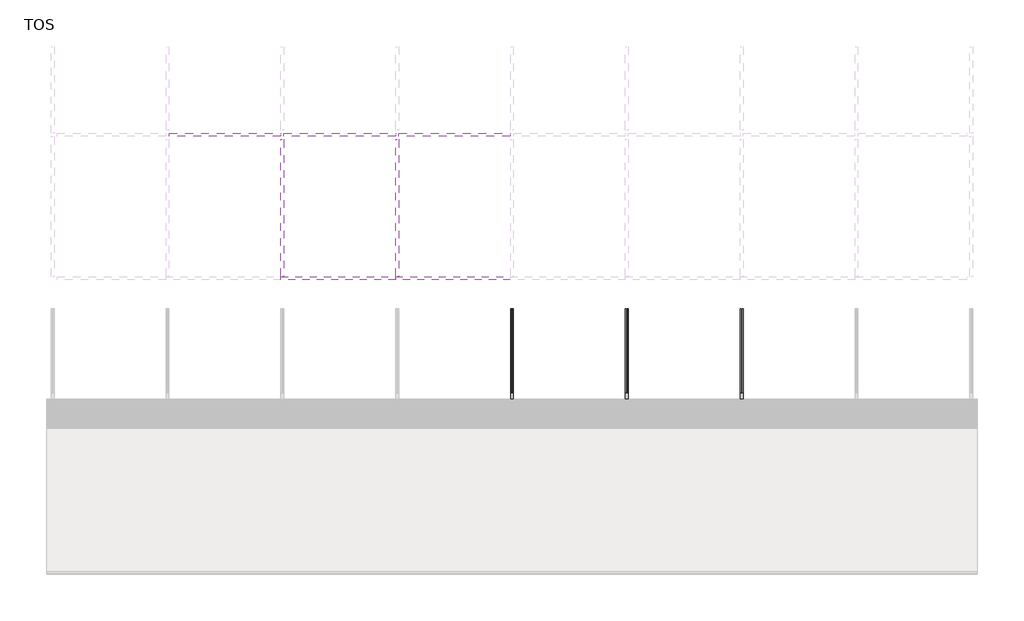
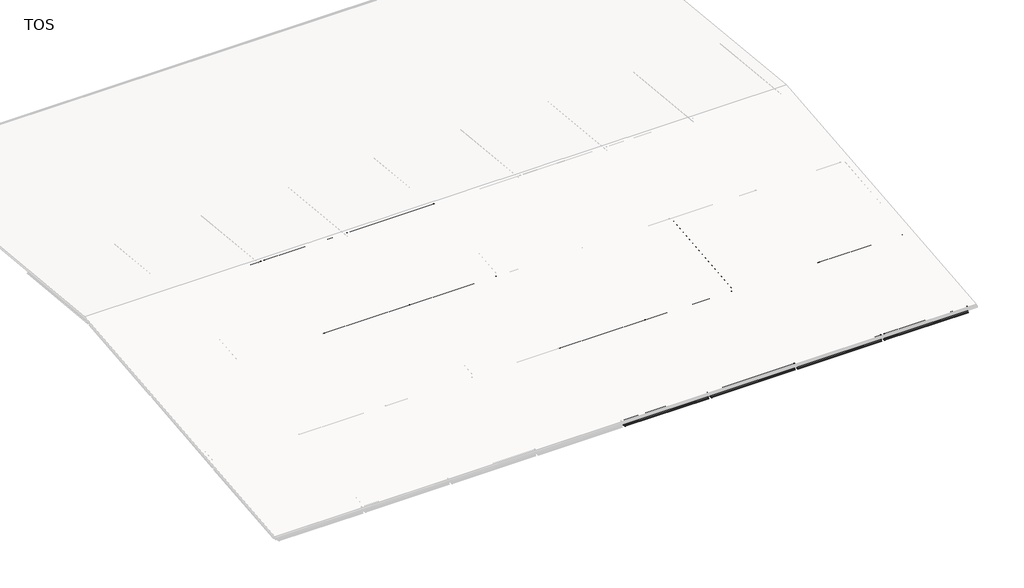
# One storey, part 2 of 5: 22 beams.
"""IFC4 building model written with IfcOpenShell, lengths in millimetres."""

import ifcopenshell
import ifcopenshell.guid

model = None  # the IFC model being written
_history = None  # IfcOwnerHistory: only IFC2X3 demands one
_inside = {}  # id of a spatial element -> (the spatial element, [elements in it])
_under = {}  # id of a project, library or spatial element -> (it, [spatial elements below it])
_declared = {}  # id of a project -> (the project, [libraries it declares])
_typed = {}  # id of a type object -> (the type object, [elements of that type])
_made_of = {}  # id of a material, layer set ... -> (it, [elements and type objects made of it])


def new_model(schema):
    """Start an empty IFC model of exactly this schema.

    Asked for "IFC4X3", IfcOpenShell would pick the latest addendum, in which some entities
    have other attributes; the version numbers below select the first issue.
    IFC2X3 requires an IfcOwnerHistory on every rooted entity: one is made here for all.
    """
    global model, _history
    if schema == "IFC4X3":
        model = ifcopenshell.file(schema_version=(4, 3, 0, 0))
    else:
        model = ifcopenshell.file(schema=schema)
    _inside.clear()
    _under.clear()
    _declared.clear()
    _typed.clear()
    _made_of.clear()
    _history = None
    if model.schema == "IFC2X3":
        org = make("IfcOrganization", Name="unknown")
        user = make(
            "IfcPersonAndOrganization",
            ThePerson=make("IfcPerson", FamilyName="unknown"),
            TheOrganization=org,
        )
        app = make(
            "IfcApplication",
            ApplicationDeveloper=org,
            Version="unknown",
            ApplicationFullName="unknown",
            ApplicationIdentifier="unknown",
        )
        _history = make(
            "IfcOwnerHistory",
            OwningUser=user,
            OwningApplication=app,
            ChangeAction="ADDED",
            CreationDate=0,
        )
    return model


def make(cls, **values):
    """One entity of the class cls with the attributes given. An attribute that is None is left unset."""
    return model.create_entity(
        cls, **{name: value for name, value in values.items() if value is not None}
    )


def rooted(cls, **values):
    """An entity with a GlobalId (a new one), such as an element, a storey or a relation."""
    return make(cls, GlobalId=ifcopenshell.guid.new(), OwnerHistory=_history, **values)


def si_unit(unit_type, name, prefix=None):
    """IfcSIUnit, for example si_unit("LENGTHUNIT", "METRE", prefix="MILLI")."""
    return make("IfcSIUnit", UnitType=unit_type, Prefix=prefix, Name=name)


def assignment(units):
    """IfcUnitAssignment: the units of a project."""
    return None if units is None else make("IfcUnitAssignment", Units=units)


def point(xyz):
    """IfcCartesianPoint."""
    return None if xyz is None else make("IfcCartesianPoint", Coordinates=xyz)


def direction(xyz):
    """IfcDirection."""
    return None if xyz is None else make("IfcDirection", DirectionRatios=xyz)


def frame(location, z_axis=None, x_axis=None):
    """IfcAxis2Placement3D, a coordinate frame: its origin and axes. An axis left out is left unset."""
    return make(
        "IfcAxis2Placement3D",
        Location=point(location),
        Axis=direction(z_axis),
        RefDirection=direction(x_axis),
    )


def frame_2d(location, x_axis=None):
    """IfcAxis2Placement2D, a coordinate frame in the plane: its origin and x axis."""
    return make(
        "IfcAxis2Placement2D", Location=point(location), RefDirection=direction(x_axis)
    )


def origin():
    """The frame at (0, 0, 0) with its axes left unset."""
    return frame((0.0, 0.0, 0.0))


def place(relative_to, where):
    """IfcLocalPlacement: puts the frame where relative to a parent placement (None: the world)."""
    return make(
        "IfcLocalPlacement", PlacementRelTo=relative_to, RelativePlacement=where
    )


def context(
    kind, dimensions, precision=None, world=None, true_north=None, identifier=None
):
    """IfcGeometricRepresentationContext, for example the 3D "Model" context."""
    return make(
        "IfcGeometricRepresentationContext",
        ContextIdentifier=identifier,
        ContextType=kind,
        CoordinateSpaceDimension=dimensions,
        Precision=precision,
        WorldCoordinateSystem=world,
        TrueNorth=true_north,
    )


def project(units=None, contexts=None):
    """IfcProject with its units and contexts."""
    return rooted(
        "IfcProject",
        Name="project",
        RepresentationContexts=contexts,
        UnitsInContext=assignment(units),
    )


def spatial(cls, under=None, at=None, **own):
    """A site, building, storey or space (cls), placed at a placement, below another one or the project."""
    s = rooted(cls, ObjectPlacement=at, **own)
    if under is not None:
        _under.setdefault(under.id(), (under, []))[1].append(s)
    return s


def polyline(points):
    """IfcPolyline through the points."""
    return make("IfcPolyline", Points=[point(p) for p in points])


def circle_curve(where, radius):
    """IfcCircle in the frame where."""
    return make("IfcCircle", Position=where, Radius=radius)


def trimmed(basis, trim1, trim2, sense, master):
    """IfcTrimmedCurve: the piece of a basis curve between two trims."""
    return make(
        "IfcTrimmedCurve",
        BasisCurve=basis,
        Trim1=trim1,
        Trim2=trim2,
        SenseAgreement=sense,
        MasterRepresentation=master,
    )


def segment(curve, same_sense, transition):
    """IfcCompositeCurveSegment."""
    return make(
        "IfcCompositeCurveSegment",
        Transition=transition,
        SameSense=same_sense,
        ParentCurve=curve,
    )


def composite_curve(segments, self_intersect=None):
    """IfcCompositeCurve: segments joined end to end."""
    return make("IfcCompositeCurve", Segments=segments, SelfIntersect=self_intersect)


def outline(outer, holes=None, kind="AREA"):
    """IfcArbitraryClosedProfileDef: a profile drawn as a closed curve; with holes, ...WithVoids."""
    if holes is None:
        return make("IfcArbitraryClosedProfileDef", ProfileType=kind, OuterCurve=outer)
    return make(
        "IfcArbitraryProfileDefWithVoids",
        ProfileType=kind,
        OuterCurve=outer,
        InnerCurves=holes,
    )


def extrude(swept, where, along, depth):
    """IfcExtrudedAreaSolid: the profile swept, set in the frame where, extruded along a direction by depth."""
    return make(
        "IfcExtrudedAreaSolid",
        SweptArea=swept,
        Position=where,
        ExtrudedDirection=direction(along),
        Depth=depth,
    )


def shape(context_of_items, identifier, shape_type, items):
    """IfcShapeRepresentation: the items that make up one representation, for example the "Body"."""
    return make(
        "IfcShapeRepresentation",
        ContextOfItems=context_of_items,
        RepresentationIdentifier=identifier,
        RepresentationType=shape_type,
        Items=items,
    )


def made_of(thing, what):
    """Note that an element or type object is made of a material, layer set ...; save() writes the relation."""
    if what is not None:
        _made_of.setdefault(what.id(), (what, []))[1].append(thing)
    return thing


def element(
    cls,
    number,
    at=None,
    inside=None,
    cuts=None,
    type_object=None,
    material=None,
    context=None,
    identifier="Body",
    shape_type=None,
    held_by="IfcProductDefinitionShape",
    body=None,
    shapes=None,
    **own,
):
    """One element of the class cls, such as IfcWall. Its Tag is "e" and its number.

    at: its placement. inside: the storey or other place that contains it. cuts: it is an
    opening in that element (IfcRelVoidsElement). A single representation is given by context,
    identifier, shape_type and body (its items); several are given by shapes. held_by: the class
    of the entity that holds the representations. save() writes the other relations.
    """
    e = rooted(cls, Tag="e%d" % number, ObjectPlacement=at, **own)
    if body is not None:
        shapes = [shape(context, identifier, shape_type, body)]
    if shapes is not None:
        e.Representation = make(held_by, Representations=shapes)
    if inside is not None:
        _inside.setdefault(inside.id(), (inside, []))[1].append(e)
    if cuts is not None:
        rooted(
            "IfcRelVoidsElement", RelatingBuildingElement=cuts, RelatedOpeningElement=e
        )
    if type_object is not None:
        _typed.setdefault(type_object.id(), (type_object, []))[1].append(e)
    return made_of(e, material)


def aggregate(whole, parts):
    """IfcRelAggregates: a whole, such as a stair, and the parts it consists of."""
    return rooted("IfcRelAggregates", RelatingObject=whole, RelatedObjects=parts)


def save(model, path):
    """Write the relations noted so far, then the file.

    IfcRelAggregates (storeys below a building ...), IfcRelContainedInSpatialStructure (elements
    in a storey), IfcRelDefinesByType, IfcRelAssociatesMaterial and IfcRelDeclares: one each for
    every whole, place, type object, material and project.
    """
    for whole, parts in _under.values():
        aggregate(whole, parts)
    for where, things in _inside.values():
        rooted(
            "IfcRelContainedInSpatialStructure",
            RelatedElements=things,
            RelatingStructure=where,
        )
    for kind, things in _typed.values():
        rooted("IfcRelDefinesByType", RelatedObjects=things, RelatingType=kind)
    for what, things in _made_of.values():
        rooted("IfcRelAssociatesMaterial", RelatedObjects=things, RelatingMaterial=what)
    for by, libraries in _declared.values():
        rooted("IfcRelDeclares", RelatingContext=by, RelatedDefinitions=libraries)
    model.write(path)


model = new_model("IFC4")

# Units and contexts
model_context = context("Model", 3, world=origin())
ifc_project = project(units=[si_unit("LENGTHUNIT", "METRE", prefix="MILLI")], contexts=[model_context])

# Site, building, storey
site = spatial("IfcSite", under=ifc_project)
building = spatial("IfcBuilding", under=site)
storey = spatial("IfcBuildingStorey", under=building, Name="TOS", Elevation=9299.9618634)

# Beams
placement = place(None, origin())
element("IfcBeam", 1, ObjectType="0912_Steel Framing_H-KSD3502 : H_SB_ASB_H-600x200x11x17", at=placement, inside=storey, context=model_context, shape_type="SweptSolid", body=[
    extrude(outline(composite_curve([segment(polyline([(10599.5208589, 9716.9618634), (10599.5208589, 9699.9618634), (10399.5208589, 9699.9618634), (10399.5208589, 9716.9618634), (10472.0208589, 9716.9618634)]), True, "CONTINUOUS"), segment(trimmed(circle_curve(frame_2d((10472.0208589, 9738.9618634)), 22.0), [point((10472.0208589, 9716.9618634))], [point((10494.0208589, 9738.9618634))], True, "CARTESIAN"), True, "CONTINUOUS"), segment(polyline([(10494.0208589, 9738.9618634), (10494.0208589, 10260.9618634)]), True, "CONTINUOUS"), segment(trimmed(circle_curve(frame_2d((10472.0208589, 10260.9618634)), 22.0), [point((10494.0208589, 10260.9618634))], [point((10472.0208589, 10282.9618634))], True, "CARTESIAN"), True, "CONTINUOUS"), segment(polyline([(10472.0208589, 10282.9618634), (10399.5208589, 10282.9618634), (10399.5208589, 10299.9618634), (10599.5208589, 10299.9618634), (10599.5208589, 10282.9618634), (10527.0208589, 10282.9618634)]), True, "CONTINUOUS"), segment(trimmed(circle_curve(frame_2d((10527.0208589, 10260.9618634)), 22.0), [point((10527.0208589, 10282.9618634))], [point((10505.0208589, 10260.9618634))], True, "CARTESIAN"), True, "CONTINUOUS"), segment(polyline([(10505.0208589, 10260.9618634), (10505.0208589, 9738.9618634)]), True, "CONTINUOUS"), segment(trimmed(circle_curve(frame_2d((10527.0208589, 9738.9618634)), 22.0), [point((10505.0208589, 9738.9618634))], [point((10527.0208589, 9716.9618634))], True, "CARTESIAN"), True, "CONTINUOUS"), segment(polyline([(10527.0208589, 9716.9618634), (10599.5208589, 9716.9618634)]), True, "CONTINUOUS")], self_intersect=False)), frame((31900.0, 0.0, 0.0), z_axis=(1.0, 0.0, 0.0), x_axis=(0.0, 1.0, 0.0)), (0.0, 0.0, 1.0), 7987.3),
])
element("IfcBeam", 2, ObjectType="0912_Steel Framing_H-KSD3502 : H_SB_ASB_H-600x200x11x17", at=placement, inside=storey, context=model_context, shape_type="SweptSolid", body=[
    extrude(outline(composite_curve([segment(polyline([(10599.5208589, 9716.9618634), (10599.5208589, 9699.9618634), (10399.5208589, 9699.9618634), (10399.5208589, 9716.9618634), (10472.0208589, 9716.9618634)]), True, "CONTINUOUS"), segment(trimmed(circle_curve(frame_2d((10472.0208589, 9738.9618634)), 22.0), [point((10472.0208589, 9716.9618634))], [point((10494.0208589, 9738.9618634))], True, "CARTESIAN"), True, "CONTINUOUS"), segment(polyline([(10494.0208589, 9738.9618634), (10494.0208589, 10260.9618634)]), True, "CONTINUOUS"), segment(trimmed(circle_curve(frame_2d((10472.0208589, 10260.9618634)), 22.0), [point((10494.0208589, 10260.9618634))], [point((10472.0208589, 10282.9618634))], True, "CARTESIAN"), True, "CONTINUOUS"), segment(polyline([(10472.0208589, 10282.9618634), (10399.5208589, 10282.9618634), (10399.5208589, 10299.9618634), (10599.5208589, 10299.9618634), (10599.5208589, 10282.9618634), (10527.0208589, 10282.9618634)]), True, "CONTINUOUS"), segment(trimmed(circle_curve(frame_2d((10527.0208589, 10260.9618634)), 22.0), [point((10527.0208589, 10282.9618634))], [point((10505.0208589, 10260.9618634))], True, "CARTESIAN"), True, "CONTINUOUS"), segment(polyline([(10505.0208589, 10260.9618634), (10505.0208589, 9738.9618634)]), True, "CONTINUOUS"), segment(trimmed(circle_curve(frame_2d((10527.0208589, 9738.9618634)), 22.0), [point((10505.0208589, 9738.9618634))], [point((10527.0208589, 9716.9618634))], True, "CARTESIAN"), True, "CONTINUOUS"), segment(polyline([(10527.0208589, 9716.9618634), (10599.5208589, 9716.9618634)]), True, "CONTINUOUS")], self_intersect=False)), frame((39900.0, 0.0, 0.0), z_axis=(1.0, 0.0, 0.0), x_axis=(0.0, 1.0, 0.0)), (0.0, 0.0, 1.0), 7987.3),
])
element("IfcBeam", 3, ObjectType="0912_Steel Framing_H-KSD3502 : H_SB_ASB_H-600x200x11x17", at=placement, inside=storey, context=model_context, shape_type="SweptSolid", body=[
    extrude(outline(composite_curve([segment(polyline([(10599.5208589, 9716.9618634), (10599.5208589, 9699.9618634), (10399.5208589, 9699.9618634), (10399.5208589, 9716.9618634), (10472.0208589, 9716.9618634)]), True, "CONTINUOUS"), segment(trimmed(circle_curve(frame_2d((10472.0208589, 9738.9618634)), 22.0), [point((10472.0208589, 9716.9618634))], [point((10494.0208589, 9738.9618634))], True, "CARTESIAN"), True, "CONTINUOUS"), segment(polyline([(10494.0208589, 9738.9618634), (10494.0208589, 10260.9618634)]), True, "CONTINUOUS"), segment(trimmed(circle_curve(frame_2d((10472.0208589, 10260.9618634)), 22.0), [point((10494.0208589, 10260.9618634))], [point((10472.0208589, 10282.9618634))], True, "CARTESIAN"), True, "CONTINUOUS"), segment(polyline([(10472.0208589, 10282.9618634), (10399.5208589, 10282.9618634), (10399.5208589, 10299.9618634), (10599.5208589, 10299.9618634), (10599.5208589, 10282.9618634), (10527.0208589, 10282.9618634)]), True, "CONTINUOUS"), segment(trimmed(circle_curve(frame_2d((10527.0208589, 10260.9618634)), 22.0), [point((10527.0208589, 10282.9618634))], [point((10505.0208589, 10260.9618634))], True, "CARTESIAN"), True, "CONTINUOUS"), segment(polyline([(10505.0208589, 10260.9618634), (10505.0208589, 9738.9618634)]), True, "CONTINUOUS"), segment(trimmed(circle_curve(frame_2d((10527.0208589, 9738.9618634)), 22.0), [point((10505.0208589, 9738.9618634))], [point((10527.0208589, 9716.9618634))], True, "CARTESIAN"), True, "CONTINUOUS"), segment(polyline([(10527.0208589, 9716.9618634), (10599.5208589, 9716.9618634)]), True, "CONTINUOUS")], self_intersect=False)), frame((47900.0, 0.0, 0.0), z_axis=(1.0, 0.0, 0.0), x_axis=(0.0, 1.0, 0.0)), (0.0, 0.0, 1.0), 7987.3),
])
element("IfcBeam", 4, ObjectType="0912_Steel Framing_H-KSD3502 : H_SB_ASB_H-600x200x11x17", at=placement, inside=storey, context=model_context, shape_type="SweptSolid", body=[
    extrude(outline(composite_curve([segment(polyline([(10599.5208589, 9716.9618634), (10599.5208589, 9699.9618634), (10399.5208589, 9699.9618634), (10399.5208589, 9716.9618634), (10472.0208589, 9716.9618634)]), True, "CONTINUOUS"), segment(trimmed(circle_curve(frame_2d((10472.0208589, 9738.9618634)), 22.0), [point((10472.0208589, 9716.9618634))], [point((10494.0208589, 9738.9618634))], True, "CARTESIAN"), True, "CONTINUOUS"), segment(polyline([(10494.0208589, 9738.9618634), (10494.0208589, 10260.9618634)]), True, "CONTINUOUS"), segment(trimmed(circle_curve(frame_2d((10472.0208589, 10260.9618634)), 22.0), [point((10494.0208589, 10260.9618634))], [point((10472.0208589, 10282.9618634))], True, "CARTESIAN"), True, "CONTINUOUS"), segment(polyline([(10472.0208589, 10282.9618634), (10399.5208589, 10282.9618634), (10399.5208589, 10299.9618634), (10599.5208589, 10299.9618634), (10599.5208589, 10282.9618634), (10527.0208589, 10282.9618634)]), True, "CONTINUOUS"), segment(trimmed(circle_curve(frame_2d((10527.0208589, 10260.9618634)), 22.0), [point((10527.0208589, 10282.9618634))], [point((10505.0208589, 10260.9618634))], True, "CARTESIAN"), True, "CONTINUOUS"), segment(polyline([(10505.0208589, 10260.9618634), (10505.0208589, 9738.9618634)]), True, "CONTINUOUS"), segment(trimmed(circle_curve(frame_2d((10527.0208589, 9738.9618634)), 22.0), [point((10505.0208589, 9738.9618634))], [point((10527.0208589, 9716.9618634))], True, "CARTESIAN"), True, "CONTINUOUS"), segment(polyline([(10527.0208589, 9716.9618634), (10599.5208589, 9716.9618634)]), True, "CONTINUOUS")], self_intersect=False)), frame((55900.0, 0.0, 0.0), z_axis=(1.0, 0.0, 0.0), x_axis=(0.0, 1.0, 0.0)), (0.0, 0.0, 1.0), 7781.3),
])
element("IfcBeam", 5, ObjectType="0912_Steel Framing_H-KSD3502 : H_SB_ASB_H-600x200x11x17", at=placement, inside=storey, context=model_context, shape_type="SweptSolid", body=[
    extrude(outline(composite_curve([segment(polyline([(599.5208589, 8716.9618634), (599.5208589, 8699.9618634), (399.5208589, 8699.9618634), (399.5208589, 8716.9618634), (472.0208589, 8716.9618634)]), True, "CONTINUOUS"), segment(trimmed(circle_curve(frame_2d((472.0208589, 8738.9618634)), 22.0), [point((472.0208589, 8716.9618634))], [point((494.0208589, 8738.9618634))], True, "CARTESIAN"), True, "CONTINUOUS"), segment(polyline([(494.0208589, 8738.9618634), (494.0208589, 9260.9618634)]), True, "CONTINUOUS"), segment(trimmed(circle_curve(frame_2d((472.0208589, 9260.9618634)), 22.0), [point((494.0208589, 9260.9618634))], [point((472.0208589, 9282.9618634))], True, "CARTESIAN"), True, "CONTINUOUS"), segment(polyline([(472.0208589, 9282.9618634), (399.5208589, 9282.9618634), (399.5208589, 9299.9618634), (599.5208589, 9299.9618634), (599.5208589, 9282.9618634), (527.0208589, 9282.9618634)]), True, "CONTINUOUS"), segment(trimmed(circle_curve(frame_2d((527.0208589, 9260.9618634)), 22.0), [point((527.0208589, 9282.9618634))], [point((505.0208589, 9260.9618634))], True, "CARTESIAN"), True, "CONTINUOUS"), segment(polyline([(505.0208589, 9260.9618634), (505.0208589, 8738.9618634)]), True, "CONTINUOUS"), segment(trimmed(circle_curve(frame_2d((527.0208589, 8738.9618634)), 22.0), [point((505.0208589, 8738.9618634))], [point((527.0208589, 8716.9618634))], True, "CARTESIAN"), True, "CONTINUOUS"), segment(polyline([(527.0208589, 8716.9618634), (599.5208589, 8716.9618634)]), True, "CONTINUOUS")], self_intersect=False)), frame((32113.7, 0.0, 0.0), z_axis=(1.0, 0.0, 0.0), x_axis=(0.0, 1.0, 0.0)), (0.0, 0.0, 1.0), 7772.6),
])
element("IfcBeam", 6, ObjectType="0912_Steel Framing_H-KSD3502 : H_SB_ASB_H-600x200x11x17", at=placement, inside=storey, context=model_context, shape_type="SweptSolid", body=[
    extrude(outline(composite_curve([segment(polyline([(599.5208589, 8716.9618634), (599.5208589, 8699.9618634), (399.5208589, 8699.9618634), (399.5208589, 8716.9618634), (472.0208589, 8716.9618634)]), True, "CONTINUOUS"), segment(trimmed(circle_curve(frame_2d((472.0208589, 8738.9618634)), 22.0), [point((472.0208589, 8716.9618634))], [point((494.0208589, 8738.9618634))], True, "CARTESIAN"), True, "CONTINUOUS"), segment(polyline([(494.0208589, 8738.9618634), (494.0208589, 9260.9618634)]), True, "CONTINUOUS"), segment(trimmed(circle_curve(frame_2d((472.0208589, 9260.9618634)), 22.0), [point((494.0208589, 9260.9618634))], [point((472.0208589, 9282.9618634))], True, "CARTESIAN"), True, "CONTINUOUS"), segment(polyline([(472.0208589, 9282.9618634), (399.5208589, 9282.9618634), (399.5208589, 9299.9618634), (599.5208589, 9299.9618634), (599.5208589, 9282.9618634), (527.0208589, 9282.9618634)]), True, "CONTINUOUS"), segment(trimmed(circle_curve(frame_2d((527.0208589, 9260.9618634)), 22.0), [point((527.0208589, 9282.9618634))], [point((505.0208589, 9260.9618634))], True, "CARTESIAN"), True, "CONTINUOUS"), segment(polyline([(505.0208589, 9260.9618634), (505.0208589, 8738.9618634)]), True, "CONTINUOUS"), segment(trimmed(circle_curve(frame_2d((527.0208589, 8738.9618634)), 22.0), [point((505.0208589, 8738.9618634))], [point((527.0208589, 8716.9618634))], True, "CARTESIAN"), True, "CONTINUOUS"), segment(polyline([(527.0208589, 8716.9618634), (599.5208589, 8716.9618634)]), True, "CONTINUOUS")], self_intersect=False)), frame((40113.7, 0.0, 0.0), z_axis=(1.0, 0.0, 0.0), x_axis=(0.0, 1.0, 0.0)), (0.0, 0.0, 1.0), 7772.6),
])
element("IfcBeam", 7, ObjectType="0912_Steel Framing_H-KSD3502 : H_SB_ASB_H-600x200x11x17", at=placement, inside=storey, context=model_context, shape_type="SweptSolid", body=[
    extrude(outline(composite_curve([segment(polyline([(599.5208589, 8716.9618634), (599.5208589, 8699.9618634), (399.5208589, 8699.9618634), (399.5208589, 8716.9618634), (472.0208589, 8716.9618634)]), True, "CONTINUOUS"), segment(trimmed(circle_curve(frame_2d((472.0208589, 8738.9618634)), 22.0), [point((472.0208589, 8716.9618634))], [point((494.0208589, 8738.9618634))], True, "CARTESIAN"), True, "CONTINUOUS"), segment(polyline([(494.0208589, 8738.9618634), (494.0208589, 9260.9618634)]), True, "CONTINUOUS"), segment(trimmed(circle_curve(frame_2d((472.0208589, 9260.9618634)), 22.0), [point((494.0208589, 9260.9618634))], [point((472.0208589, 9282.9618634))], True, "CARTESIAN"), True, "CONTINUOUS"), segment(polyline([(472.0208589, 9282.9618634), (399.5208589, 9282.9618634), (399.5208589, 9299.9618634), (599.5208589, 9299.9618634), (599.5208589, 9282.9618634), (527.0208589, 9282.9618634)]), True, "CONTINUOUS"), segment(trimmed(circle_curve(frame_2d((527.0208589, 9260.9618634)), 22.0), [point((527.0208589, 9282.9618634))], [point((505.0208589, 9260.9618634))], True, "CARTESIAN"), True, "CONTINUOUS"), segment(polyline([(505.0208589, 9260.9618634), (505.0208589, 8738.9618634)]), True, "CONTINUOUS"), segment(trimmed(circle_curve(frame_2d((527.0208589, 8738.9618634)), 22.0), [point((505.0208589, 8738.9618634))], [point((527.0208589, 8716.9618634))], True, "CARTESIAN"), True, "CONTINUOUS"), segment(polyline([(527.0208589, 8716.9618634), (599.5208589, 8716.9618634)]), True, "CONTINUOUS")], self_intersect=False)), frame((48113.7, 0.0, 0.0), z_axis=(1.0, 0.0, 0.0), x_axis=(0.0, 1.0, 0.0)), (0.0, 0.0, 1.0), 7772.6),
])
element("IfcBeam", 8, ObjectType="0912_Steel Framing_H-KSD3502 : H_SB_ASB_H-600x200x11x17", at=placement, inside=storey, context=model_context, shape_type="SweptSolid", body=[
    extrude(outline(composite_curve([segment(polyline([(599.5208589, 8716.9618634), (599.5208589, 8699.9618634), (399.5208589, 8699.9618634), (399.5208589, 8716.9618634), (472.0208589, 8716.9618634)]), True, "CONTINUOUS"), segment(trimmed(circle_curve(frame_2d((472.0208589, 8738.9618634)), 22.0), [point((472.0208589, 8716.9618634))], [point((494.0208589, 8738.9618634))], True, "CARTESIAN"), True, "CONTINUOUS"), segment(polyline([(494.0208589, 8738.9618634), (494.0208589, 9260.9618634)]), True, "CONTINUOUS"), segment(trimmed(circle_curve(frame_2d((472.0208589, 9260.9618634)), 22.0), [point((494.0208589, 9260.9618634))], [point((472.0208589, 9282.9618634))], True, "CARTESIAN"), True, "CONTINUOUS"), segment(polyline([(472.0208589, 9282.9618634), (399.5208589, 9282.9618634), (399.5208589, 9299.9618634), (599.5208589, 9299.9618634), (599.5208589, 9282.9618634), (527.0208589, 9282.9618634)]), True, "CONTINUOUS"), segment(trimmed(circle_curve(frame_2d((527.0208589, 9260.9618634)), 22.0), [point((527.0208589, 9282.9618634))], [point((505.0208589, 9260.9618634))], True, "CARTESIAN"), True, "CONTINUOUS"), segment(polyline([(505.0208589, 9260.9618634), (505.0208589, 8738.9618634)]), True, "CONTINUOUS"), segment(trimmed(circle_curve(frame_2d((527.0208589, 8738.9618634)), 22.0), [point((505.0208589, 8738.9618634))], [point((527.0208589, 8716.9618634))], True, "CARTESIAN"), True, "CONTINUOUS"), segment(polyline([(527.0208589, 8716.9618634), (599.5208589, 8716.9618634)]), True, "CONTINUOUS")], self_intersect=False)), frame((56113.7, 0.0, 0.0), z_axis=(1.0, 0.0, 0.0), x_axis=(0.0, 1.0, 0.0)), (0.0, 0.0, 1.0), 7772.6),
])
element("IfcBeam", 9, ObjectType="0912_Steel Framing_H-KSD3502 : H_SB_ASB_H-600x200x11x17", at=placement, inside=storey, context=model_context, shape_type="SweptSolid", body=[
    extrude(outline(composite_curve([segment(polyline([(20599.5208589, 10716.9618634), (20599.5208589, 10699.9618634), (20399.5208589, 10699.9618634), (20399.5208589, 10716.9618634), (20472.0208589, 10716.9618634)]), True, "CONTINUOUS"), segment(trimmed(circle_curve(frame_2d((20472.0208589, 10738.9618634)), 22.0), [point((20472.0208589, 10716.9618634))], [point((20494.0208589, 10738.9618634))], True, "CARTESIAN"), True, "CONTINUOUS"), segment(polyline([(20494.0208589, 10738.9618634), (20494.0208589, 11260.9618634)]), True, "CONTINUOUS"), segment(trimmed(circle_curve(frame_2d((20472.0208589, 11260.9618634)), 22.0), [point((20494.0208589, 11260.9618634))], [point((20472.0208589, 11282.9618634))], True, "CARTESIAN"), True, "CONTINUOUS"), segment(polyline([(20472.0208589, 11282.9618634), (20399.5208589, 11282.9618634), (20399.5208589, 11299.9618634), (20599.5208589, 11299.9618634), (20599.5208589, 11282.9618634), (20527.0208589, 11282.9618634)]), True, "CONTINUOUS"), segment(trimmed(circle_curve(frame_2d((20527.0208589, 11260.9618634)), 22.0), [point((20527.0208589, 11282.9618634))], [point((20505.0208589, 11260.9618634))], True, "CARTESIAN"), True, "CONTINUOUS"), segment(polyline([(20505.0208589, 11260.9618634), (20505.0208589, 10738.9618634)]), True, "CONTINUOUS"), segment(trimmed(circle_curve(frame_2d((20527.0208589, 10738.9618634)), 22.0), [point((20505.0208589, 10738.9618634))], [point((20527.0208589, 10716.9618634))], True, "CARTESIAN"), True, "CONTINUOUS"), segment(polyline([(20527.0208589, 10716.9618634), (20599.5208589, 10716.9618634)]), True, "CONTINUOUS")], self_intersect=False)), frame((15900.0, 0.0, 0.0), z_axis=(1.0, 0.0, 0.0), x_axis=(0.0, 1.0, 0.0)), (0.0, 0.0, 1.0), 7987.3),
])
element("IfcBeam", 10, ObjectType="0912_Steel Framing_H-KSD3502 : H_SB_ASB_H-600x200x11x17", at=placement, inside=storey, context=model_context, shape_type="SweptSolid", body=[
    extrude(outline(composite_curve([segment(polyline([(20599.5208589, 10716.9618634), (20599.5208589, 10699.9618634), (20399.5208589, 10699.9618634), (20399.5208589, 10716.9618634), (20472.0208589, 10716.9618634)]), True, "CONTINUOUS"), segment(trimmed(circle_curve(frame_2d((20472.0208589, 10738.9618634)), 22.0), [point((20472.0208589, 10716.9618634))], [point((20494.0208589, 10738.9618634))], True, "CARTESIAN"), True, "CONTINUOUS"), segment(polyline([(20494.0208589, 10738.9618634), (20494.0208589, 11260.9618634)]), True, "CONTINUOUS"), segment(trimmed(circle_curve(frame_2d((20472.0208589, 11260.9618634)), 22.0), [point((20494.0208589, 11260.9618634))], [point((20472.0208589, 11282.9618634))], True, "CARTESIAN"), True, "CONTINUOUS"), segment(polyline([(20472.0208589, 11282.9618634), (20399.5208589, 11282.9618634), (20399.5208589, 11299.9618634), (20599.5208589, 11299.9618634), (20599.5208589, 11282.9618634), (20527.0208589, 11282.9618634)]), True, "CONTINUOUS"), segment(trimmed(circle_curve(frame_2d((20527.0208589, 11260.9618634)), 22.0), [point((20527.0208589, 11282.9618634))], [point((20505.0208589, 11260.9618634))], True, "CARTESIAN"), True, "CONTINUOUS"), segment(polyline([(20505.0208589, 11260.9618634), (20505.0208589, 10738.9618634)]), True, "CONTINUOUS"), segment(trimmed(circle_curve(frame_2d((20527.0208589, 10738.9618634)), 22.0), [point((20505.0208589, 10738.9618634))], [point((20527.0208589, 10716.9618634))], True, "CARTESIAN"), True, "CONTINUOUS"), segment(polyline([(20527.0208589, 10716.9618634), (20599.5208589, 10716.9618634)]), True, "CONTINUOUS")], self_intersect=False)), frame((23900.0, 0.0, 0.0), z_axis=(1.0, 0.0, 0.0), x_axis=(0.0, 1.0, 0.0)), (0.0, 0.0, 1.0), 7987.3),
])
element("IfcBeam", 11, ObjectType="0912_Steel Framing_H-KSD3502 : H_SB_ASB_H-600x200x11x17", at=placement, inside=storey, context=model_context, shape_type="SweptSolid", body=[
    extrude(outline(composite_curve([segment(polyline([(30599.5208589, 11716.9618634), (30599.5208589, 11699.9618634), (30399.5208589, 11699.9618634), (30399.5208589, 11716.9618634), (30472.0208589, 11716.9618634)]), True, "CONTINUOUS"), segment(trimmed(circle_curve(frame_2d((30472.0208589, 11738.9618634)), 22.0), [point((30472.0208589, 11716.9618634))], [point((30494.0208589, 11738.9618634))], True, "CARTESIAN"), True, "CONTINUOUS"), segment(polyline([(30494.0208589, 11738.9618634), (30494.0208589, 12260.9618634)]), True, "CONTINUOUS"), segment(trimmed(circle_curve(frame_2d((30472.0208589, 12260.9618634)), 22.0), [point((30494.0208589, 12260.9618634))], [point((30472.0208589, 12282.9618634))], True, "CARTESIAN"), True, "CONTINUOUS"), segment(polyline([(30472.0208589, 12282.9618634), (30399.5208589, 12282.9618634), (30399.5208589, 12299.9618634), (30599.5208589, 12299.9618634), (30599.5208589, 12282.9618634), (30527.0208589, 12282.9618634)]), True, "CONTINUOUS"), segment(trimmed(circle_curve(frame_2d((30527.0208589, 12260.9618634)), 22.0), [point((30527.0208589, 12282.9618634))], [point((30505.0208589, 12260.9618634))], True, "CARTESIAN"), True, "CONTINUOUS"), segment(polyline([(30505.0208589, 12260.9618634), (30505.0208589, 11738.9618634)]), True, "CONTINUOUS"), segment(trimmed(circle_curve(frame_2d((30527.0208589, 11738.9618634)), 22.0), [point((30505.0208589, 11738.9618634))], [point((30527.0208589, 11716.9618634))], True, "CARTESIAN"), True, "CONTINUOUS"), segment(polyline([(30527.0208589, 11716.9618634), (30599.5208589, 11716.9618634)]), True, "CONTINUOUS")], self_intersect=False)), frame((8113.7, 0.0, 0.0), z_axis=(1.0, 0.0, 0.0), x_axis=(0.0, 1.0, 0.0)), (0.0, 0.0, 1.0), 7772.6),
])
element("IfcBeam", 12, ObjectType="0912_Steel Framing_H-KSD3502 : H_SB_ASB_H-600x200x11x17", at=placement, inside=storey, context=model_context, shape_type="SweptSolid", body=[
    extrude(outline(composite_curve([segment(polyline([(30599.5208589, 11716.9618634), (30599.5208589, 11699.9618634), (30399.5208589, 11699.9618634), (30399.5208589, 11716.9618634), (30472.0208589, 11716.9618634)]), True, "CONTINUOUS"), segment(trimmed(circle_curve(frame_2d((30472.0208589, 11738.9618634)), 22.0), [point((30472.0208589, 11716.9618634))], [point((30494.0208589, 11738.9618634))], True, "CARTESIAN"), True, "CONTINUOUS"), segment(polyline([(30494.0208589, 11738.9618634), (30494.0208589, 12260.9618634)]), True, "CONTINUOUS"), segment(trimmed(circle_curve(frame_2d((30472.0208589, 12260.9618634)), 22.0), [point((30494.0208589, 12260.9618634))], [point((30472.0208589, 12282.9618634))], True, "CARTESIAN"), True, "CONTINUOUS"), segment(polyline([(30472.0208589, 12282.9618634), (30399.5208589, 12282.9618634), (30399.5208589, 12299.9618634), (30599.5208589, 12299.9618634), (30599.5208589, 12282.9618634), (30527.0208589, 12282.9618634)]), True, "CONTINUOUS"), segment(trimmed(circle_curve(frame_2d((30527.0208589, 12260.9618634)), 22.0), [point((30527.0208589, 12282.9618634))], [point((30505.0208589, 12260.9618634))], True, "CARTESIAN"), True, "CONTINUOUS"), segment(polyline([(30505.0208589, 12260.9618634), (30505.0208589, 11738.9618634)]), True, "CONTINUOUS"), segment(trimmed(circle_curve(frame_2d((30527.0208589, 11738.9618634)), 22.0), [point((30505.0208589, 11738.9618634))], [point((30527.0208589, 11716.9618634))], True, "CARTESIAN"), True, "CONTINUOUS"), segment(polyline([(30527.0208589, 11716.9618634), (30599.5208589, 11716.9618634)]), True, "CONTINUOUS")], self_intersect=False)), frame((16113.7, 0.0, 0.0), z_axis=(1.0, 0.0, 0.0), x_axis=(0.0, 1.0, 0.0)), (0.0, 0.0, 1.0), 7772.6),
])
element("IfcBeam", 13, ObjectType="0912_Steel Framing_H-KSD3502 : H_SB_ASB_H-600x200x11x17", at=placement, inside=storey, context=model_context, shape_type="SweptSolid", body=[
    extrude(outline(composite_curve([segment(polyline([(30599.5208589, 11716.9618634), (30599.5208589, 11699.9618634), (30399.5208589, 11699.9618634), (30399.5208589, 11716.9618634), (30472.0208589, 11716.9618634)]), True, "CONTINUOUS"), segment(trimmed(circle_curve(frame_2d((30472.0208589, 11738.9618634)), 22.0), [point((30472.0208589, 11716.9618634))], [point((30494.0208589, 11738.9618634))], True, "CARTESIAN"), True, "CONTINUOUS"), segment(polyline([(30494.0208589, 11738.9618634), (30494.0208589, 12260.9618634)]), True, "CONTINUOUS"), segment(trimmed(circle_curve(frame_2d((30472.0208589, 12260.9618634)), 22.0), [point((30494.0208589, 12260.9618634))], [point((30472.0208589, 12282.9618634))], True, "CARTESIAN"), True, "CONTINUOUS"), segment(polyline([(30472.0208589, 12282.9618634), (30399.5208589, 12282.9618634), (30399.5208589, 12299.9618634), (30599.5208589, 12299.9618634), (30599.5208589, 12282.9618634), (30527.0208589, 12282.9618634)]), True, "CONTINUOUS"), segment(trimmed(circle_curve(frame_2d((30527.0208589, 12260.9618634)), 22.0), [point((30527.0208589, 12282.9618634))], [point((30505.0208589, 12260.9618634))], True, "CARTESIAN"), True, "CONTINUOUS"), segment(polyline([(30505.0208589, 12260.9618634), (30505.0208589, 11738.9618634)]), True, "CONTINUOUS"), segment(trimmed(circle_curve(frame_2d((30527.0208589, 11738.9618634)), 22.0), [point((30505.0208589, 11738.9618634))], [point((30527.0208589, 11716.9618634))], True, "CARTESIAN"), True, "CONTINUOUS"), segment(polyline([(30527.0208589, 11716.9618634), (30599.5208589, 11716.9618634)]), True, "CONTINUOUS")], self_intersect=False)), frame((24113.7, 0.0, 0.0), z_axis=(1.0, 0.0, 0.0), x_axis=(0.0, 1.0, 0.0)), (0.0, 0.0, 1.0), 7772.6),
])
element("IfcBeam", 14, ObjectType="0912_Steel Framing_H-KSD3502 : H_SB_ASB_H-600x200x11x17", at=placement, inside=storey, context=model_context, shape_type="SweptSolid", body=[
    extrude(outline(composite_curve([segment(polyline([(-283.0, -100.0), (-299.9999999, -100.0), (-299.9999999, 100.0), (-283.0, 100.0), (-283.0, 27.5)]), True, "CONTINUOUS"), segment(trimmed(circle_curve(frame_2d((-261.0, 27.5)), 22.0), [point((-283.0, 27.5))], [point((-261.0, 5.5))], True, "CARTESIAN"), True, "CONTINUOUS"), segment(polyline([(-261.0, 5.5), (261.0000001, 5.5)]), True, "CONTINUOUS"), segment(trimmed(circle_curve(frame_2d((261.0000001, 27.5)), 22.0), [point((261.0000001, 5.5))], [point((283.0000001, 27.5))], True, "CARTESIAN"), True, "CONTINUOUS"), segment(polyline([(283.0000001, 27.5), (283.0000001, 100.0), (300.0, 100.0), (300.0, -100.0), (283.0000001, -100.0), (283.0000001, -27.5)]), True, "CONTINUOUS"), segment(trimmed(circle_curve(frame_2d((261.0000001, -27.5)), 22.0), [point((283.0000001, -27.5))], [point((261.0000001, -5.5))], True, "CARTESIAN"), True, "CONTINUOUS"), segment(polyline([(261.0000001, -5.5), (-261.0, -5.5)]), True, "CONTINUOUS"), segment(trimmed(circle_curve(frame_2d((-261.0, -27.5)), 22.0), [point((-261.0, -5.5))], [point((-283.0, -27.5))], True, "CARTESIAN"), True, "CONTINUOUS"), segment(polyline([(-283.0, -27.5), (-283.0, -100.0)]), True, "CONTINUOUS")], self_intersect=False)), frame((16000.0, 20641.0188479, 11012.6153936), z_axis=(0.0, 0.9950371902099892, 0.09950371902099896), x_axis=(0.0, -0.09950371902099896, 0.9950371902099892)), (0.0, 0.0, 1.0), 9557.4457081),
])
element("IfcBeam", 15, ObjectType="0912_Steel Framing_H-KSD3502 : H_SB_ASB_H-600x200x11x17", at=placement, inside=storey, context=model_context, shape_type="SweptSolid", body=[
    extrude(outline(composite_curve([segment(polyline([(-283.0, -100.0), (-299.9999999, -100.0), (-299.9999999, 100.0), (-283.0, 100.0), (-283.0, 27.5)]), True, "CONTINUOUS"), segment(trimmed(circle_curve(frame_2d((-261.0, 27.5)), 22.0), [point((-283.0, 27.5))], [point((-261.0, 5.5))], True, "CARTESIAN"), True, "CONTINUOUS"), segment(polyline([(-261.0, 5.5), (261.0000001, 5.5)]), True, "CONTINUOUS"), segment(trimmed(circle_curve(frame_2d((261.0000001, 27.5)), 22.0), [point((261.0000001, 5.5))], [point((283.0000001, 27.5))], True, "CARTESIAN"), True, "CONTINUOUS"), segment(polyline([(283.0000001, 27.5), (283.0000001, 100.0), (300.0, 100.0), (300.0, -100.0), (283.0000001, -100.0), (283.0000001, -27.5)]), True, "CONTINUOUS"), segment(trimmed(circle_curve(frame_2d((261.0000001, -27.5)), 22.0), [point((283.0000001, -27.5))], [point((261.0000001, -5.5))], True, "CARTESIAN"), True, "CONTINUOUS"), segment(polyline([(261.0000001, -5.5), (-261.0, -5.5)]), True, "CONTINUOUS"), segment(trimmed(circle_curve(frame_2d((-261.0, -27.5)), 22.0), [point((-261.0, -5.5))], [point((-283.0, -27.5))], True, "CARTESIAN"), True, "CONTINUOUS"), segment(polyline([(-283.0, -27.5), (-283.0, -100.0)]), True, "CONTINUOUS")], self_intersect=False)), frame((24000.0, 20641.0188479, 11012.6153936), z_axis=(0.0, 0.9950371902099892, 0.09950371902099887), x_axis=(0.0, -0.09950371902099887, 0.9950371902099892)), (0.0, 0.0, 1.0), 9557.4457081),
])
element("IfcBeam", 16, ObjectType="0912_Steel Framing_H-KSD3502 : H_SB_ASB_H-600x200x11x17", at=placement, inside=storey, context=model_context, shape_type="SweptSolid", body=[
    extrude(outline(composite_curve([segment(polyline([(-283.0, -100.0), (-299.9999999, -100.0), (-299.9999999, 100.0), (-283.0, 100.0), (-283.0, 27.5)]), True, "CONTINUOUS"), segment(trimmed(circle_curve(frame_2d((-261.0, 27.5)), 22.0), [point((-283.0, 27.5))], [point((-261.0, 5.5))], True, "CARTESIAN"), True, "CONTINUOUS"), segment(polyline([(-261.0, 5.5), (261.0, 5.5)]), True, "CONTINUOUS"), segment(trimmed(circle_curve(frame_2d((261.0, 27.5)), 22.0), [point((261.0, 5.5))], [point((283.0000001, 27.5))], True, "CARTESIAN"), True, "CONTINUOUS"), segment(polyline([(283.0000001, 27.5), (283.0000001, 100.0), (300.0, 100.0), (300.0, -100.0), (283.0000001, -100.0), (283.0000001, -27.5)]), True, "CONTINUOUS"), segment(trimmed(circle_curve(frame_2d((261.0, -27.5)), 22.0), [point((283.0000001, -27.5))], [point((261.0, -5.5))], True, "CARTESIAN"), True, "CONTINUOUS"), segment(polyline([(261.0, -5.5), (-261.0, -5.5)]), True, "CONTINUOUS"), segment(trimmed(circle_curve(frame_2d((-261.0, -27.5)), 22.0), [point((-261.0, -5.5))], [point((-283.0, -27.5))], True, "CARTESIAN"), True, "CONTINUOUS"), segment(polyline([(-283.0, -27.5), (-283.0, -100.0)]), True, "CONTINUOUS")], self_intersect=False)), frame((32000.0, 844.9792439, 9033.0114332), z_axis=(0.0, 0.9950371902099892, 0.09950371902099892), x_axis=(0.0, -0.09950371902099892, 0.9950371902099892)), (0.0, 0.0, 1.0), 9560.7882905),
])
element("IfcBeam", 17, ObjectType="0912_Steel Framing_H-KSD3502 : H_SB_ASB_H-600x200x11x17", at=placement, inside=storey, context=model_context, shape_type="SweptSolid", body=[
    extrude(outline(composite_curve([segment(polyline([(-283.0, -100.0), (-299.9999999, -100.0), (-299.9999999, 100.0), (-283.0, 100.0), (-283.0, 27.5)]), True, "CONTINUOUS"), segment(trimmed(circle_curve(frame_2d((-261.0, 27.5)), 22.0), [point((-283.0, 27.5))], [point((-261.0, 5.5))], True, "CARTESIAN"), True, "CONTINUOUS"), segment(polyline([(-261.0, 5.5), (261.0000001, 5.5)]), True, "CONTINUOUS"), segment(trimmed(circle_curve(frame_2d((261.0000001, 27.5)), 22.0), [point((261.0000001, 5.5))], [point((283.0000001, 27.5))], True, "CARTESIAN"), True, "CONTINUOUS"), segment(polyline([(283.0000001, 27.5), (283.0000001, 100.0), (300.0, 100.0), (300.0, -100.0), (283.0000001, -100.0), (283.0000001, -27.5)]), True, "CONTINUOUS"), segment(trimmed(circle_curve(frame_2d((261.0000001, -27.5)), 22.0), [point((283.0000001, -27.5))], [point((261.0000001, -5.5))], True, "CARTESIAN"), True, "CONTINUOUS"), segment(polyline([(261.0000001, -5.5), (-261.0, -5.5)]), True, "CONTINUOUS"), segment(trimmed(circle_curve(frame_2d((-261.0, -27.5)), 22.0), [point((-261.0, -5.5))], [point((-283.0, -27.5))], True, "CARTESIAN"), True, "CONTINUOUS"), segment(polyline([(-283.0, -27.5), (-283.0, -100.0)]), True, "CONTINUOUS")], self_intersect=False)), frame((32000.0, 10641.0188479, 10012.6153936), z_axis=(0.0, 0.9950371902099892, 0.09950371902099894), x_axis=(0.0, -0.09950371902099894, 0.9950371902099892)), (0.0, 0.0, 1.0), 9765.7659517),
])
element("IfcBeam", 18, ObjectType="0912_Steel Framing_H-KSD3502 : H_SB_ASB_H-600x200x11x17", at=placement, inside=storey, context=model_context, shape_type="SweptSolid", body=[
    extrude(outline(composite_curve([segment(polyline([(-283.0, -100.0), (-299.9999999, -100.0), (-299.9999999, 100.0), (-283.0, 100.0), (-283.0, 27.5)]), True, "CONTINUOUS"), segment(trimmed(circle_curve(frame_2d((-261.0, 27.5)), 22.0), [point((-283.0, 27.5))], [point((-261.0, 5.5))], True, "CARTESIAN"), True, "CONTINUOUS"), segment(polyline([(-261.0, 5.5), (261.0, 5.5)]), True, "CONTINUOUS"), segment(trimmed(circle_curve(frame_2d((261.0, 27.5)), 22.0), [point((261.0, 5.5))], [point((283.0000001, 27.5))], True, "CARTESIAN"), True, "CONTINUOUS"), segment(polyline([(283.0000001, 27.5), (283.0000001, 100.0), (300.0, 100.0), (300.0, -100.0), (283.0000001, -100.0), (283.0000001, -27.5)]), True, "CONTINUOUS"), segment(trimmed(circle_curve(frame_2d((261.0, -27.5)), 22.0), [point((283.0000001, -27.5))], [point((261.0, -5.5))], True, "CARTESIAN"), True, "CONTINUOUS"), segment(polyline([(261.0, -5.5), (-261.0, -5.5)]), True, "CONTINUOUS"), segment(trimmed(circle_curve(frame_2d((-261.0, -27.5)), 22.0), [point((-261.0, -5.5))], [point((-283.0, -27.5))], True, "CARTESIAN"), True, "CONTINUOUS"), segment(polyline([(-283.0, -27.5), (-283.0, -100.0)]), True, "CONTINUOUS")], self_intersect=False)), frame((40000.0, 844.9792439, 9033.0114332), z_axis=(0.0, 0.9950371902099892, 0.09950371902099892), x_axis=(0.0, -0.09950371902099892, 0.9950371902099892)), (0.0, 0.0, 1.0), 9560.7882905),
])
element("IfcBeam", 19, ObjectType="0912_Steel Framing_H-KSD3502 : H_SB_ASB_H-600x200x11x17", at=placement, inside=storey, context=model_context, shape_type="SweptSolid", body=[
    extrude(outline(composite_curve([segment(polyline([(-283.0, -100.0), (-299.9999999, -100.0), (-299.9999999, 100.0), (-283.0, 100.0), (-283.0, 27.5)]), True, "CONTINUOUS"), segment(trimmed(circle_curve(frame_2d((-261.0, 27.5)), 22.0), [point((-283.0, 27.5))], [point((-261.0, 5.5))], True, "CARTESIAN"), True, "CONTINUOUS"), segment(polyline([(-261.0, 5.5), (261.0000001, 5.5)]), True, "CONTINUOUS"), segment(trimmed(circle_curve(frame_2d((261.0000001, 27.5)), 22.0), [point((261.0000001, 5.5))], [point((283.0000001, 27.5))], True, "CARTESIAN"), True, "CONTINUOUS"), segment(polyline([(283.0000001, 27.5), (283.0000001, 100.0), (300.0, 100.0), (300.0, -100.0), (283.0000001, -100.0), (283.0000001, -27.5)]), True, "CONTINUOUS"), segment(trimmed(circle_curve(frame_2d((261.0000001, -27.5)), 22.0), [point((283.0000001, -27.5))], [point((261.0000001, -5.5))], True, "CARTESIAN"), True, "CONTINUOUS"), segment(polyline([(261.0000001, -5.5), (-261.0, -5.5)]), True, "CONTINUOUS"), segment(trimmed(circle_curve(frame_2d((-261.0, -27.5)), 22.0), [point((-261.0, -5.5))], [point((-283.0, -27.5))], True, "CARTESIAN"), True, "CONTINUOUS"), segment(polyline([(-283.0, -27.5), (-283.0, -100.0)]), True, "CONTINUOUS")], self_intersect=False)), frame((40000.0, 10641.0188479, 10012.6153936), z_axis=(0.0, 0.9950371902099892, 0.09950371902099894), x_axis=(0.0, -0.09950371902099894, 0.9950371902099892)), (0.0, 0.0, 1.0), 9765.7659517),
])
element("IfcBeam", 20, ObjectType="0912_Steel Framing_H-KSD3502 : H_SB_ASB_H-600x200x11x17", at=placement, inside=storey, context=model_context, shape_type="SweptSolid", body=[
    extrude(outline(composite_curve([segment(polyline([(-283.0, -100.0), (-299.9999999, -100.0), (-299.9999999, 100.0), (-283.0, 100.0), (-283.0, 27.5)]), True, "CONTINUOUS"), segment(trimmed(circle_curve(frame_2d((-261.0, 27.5)), 22.0), [point((-283.0, 27.5))], [point((-261.0, 5.5))], True, "CARTESIAN"), True, "CONTINUOUS"), segment(polyline([(-261.0, 5.5), (261.0, 5.5)]), True, "CONTINUOUS"), segment(trimmed(circle_curve(frame_2d((261.0, 27.5)), 22.0), [point((261.0, 5.5))], [point((283.0000001, 27.5))], True, "CARTESIAN"), True, "CONTINUOUS"), segment(polyline([(283.0000001, 27.5), (283.0000001, 100.0), (300.0, 100.0), (300.0, -100.0), (283.0000001, -100.0), (283.0000001, -27.5)]), True, "CONTINUOUS"), segment(trimmed(circle_curve(frame_2d((261.0, -27.5)), 22.0), [point((283.0000001, -27.5))], [point((261.0, -5.5))], True, "CARTESIAN"), True, "CONTINUOUS"), segment(polyline([(261.0, -5.5), (-261.0, -5.5)]), True, "CONTINUOUS"), segment(trimmed(circle_curve(frame_2d((-261.0, -27.5)), 22.0), [point((-261.0, -5.5))], [point((-283.0, -27.5))], True, "CARTESIAN"), True, "CONTINUOUS"), segment(polyline([(-283.0, -27.5), (-283.0, -100.0)]), True, "CONTINUOUS")], self_intersect=False)), frame((48000.0, 844.9792439, 9033.0114332), z_axis=(0.0, 0.9950371902099892, 0.09950371902099892), x_axis=(0.0, -0.09950371902099892, 0.9950371902099892)), (0.0, 0.0, 1.0), 9560.7882905),
])
element("IfcBeam", 21, ObjectType="0912_Steel Framing_H-KSD3502 : H_SB_ASB_H-600x200x11x17", at=placement, inside=storey, context=model_context, shape_type="SweptSolid", body=[
    extrude(outline(composite_curve([segment(polyline([(-283.0, -100.0), (-299.9999999, -100.0), (-299.9999999, 100.0), (-283.0, 100.0), (-283.0, 27.5)]), True, "CONTINUOUS"), segment(trimmed(circle_curve(frame_2d((-261.0, 27.5)), 22.0), [point((-283.0, 27.5))], [point((-261.0, 5.5))], True, "CARTESIAN"), True, "CONTINUOUS"), segment(polyline([(-261.0, 5.5), (261.0000001, 5.5)]), True, "CONTINUOUS"), segment(trimmed(circle_curve(frame_2d((261.0000001, 27.5)), 22.0), [point((261.0000001, 5.5))], [point((283.0000001, 27.5))], True, "CARTESIAN"), True, "CONTINUOUS"), segment(polyline([(283.0000001, 27.5), (283.0000001, 100.0), (300.0, 100.0), (300.0, -100.0), (283.0000001, -100.0), (283.0000001, -27.5)]), True, "CONTINUOUS"), segment(trimmed(circle_curve(frame_2d((261.0000001, -27.5)), 22.0), [point((283.0000001, -27.5))], [point((261.0000001, -5.5))], True, "CARTESIAN"), True, "CONTINUOUS"), segment(polyline([(261.0000001, -5.5), (-261.0, -5.5)]), True, "CONTINUOUS"), segment(trimmed(circle_curve(frame_2d((-261.0, -27.5)), 22.0), [point((-261.0, -5.5))], [point((-283.0, -27.5))], True, "CARTESIAN"), True, "CONTINUOUS"), segment(polyline([(-283.0, -27.5), (-283.0, -100.0)]), True, "CONTINUOUS")], self_intersect=False)), frame((48000.0, 10641.0188479, 10012.6153936), z_axis=(0.0, 0.9950371902099892, 0.09950371902099894), x_axis=(0.0, -0.09950371902099894, 0.9950371902099892)), (0.0, 0.0, 1.0), 9765.7659517),
])
element("IfcBeam", 22, ObjectType="0912_Steel Framing_H-KSD3502 : H_SB_ASB_H-600x200x11x17", at=placement, inside=storey, context=model_context, shape_type="SweptSolid", body=[
    extrude(outline(composite_curve([segment(polyline([(-283.0, -100.0), (-299.9999999, -100.0), (-299.9999999, 100.0), (-283.0, 100.0), (-283.0, 27.5)]), True, "CONTINUOUS"), segment(trimmed(circle_curve(frame_2d((-261.0, 27.5)), 22.0), [point((-283.0, 27.5))], [point((-261.0, 5.5))], True, "CARTESIAN"), True, "CONTINUOUS"), segment(polyline([(-261.0, 5.5), (261.0, 5.5)]), True, "CONTINUOUS"), segment(trimmed(circle_curve(frame_2d((261.0, 27.5)), 22.0), [point((261.0, 5.5))], [point((283.0000001, 27.5))], True, "CARTESIAN"), True, "CONTINUOUS"), segment(polyline([(283.0000001, 27.5), (283.0000001, 100.0), (300.0, 100.0), (300.0, -100.0), (283.0000001, -100.0), (283.0000001, -27.5)]), True, "CONTINUOUS"), segment(trimmed(circle_curve(frame_2d((261.0, -27.5)), 22.0), [point((283.0000001, -27.5))], [point((261.0, -5.5))], True, "CARTESIAN"), True, "CONTINUOUS"), segment(polyline([(261.0, -5.5), (-261.0, -5.5)]), True, "CONTINUOUS"), segment(trimmed(circle_curve(frame_2d((-261.0, -27.5)), 22.0), [point((-261.0, -5.5))], [point((-283.0, -27.5))], True, "CARTESIAN"), True, "CONTINUOUS"), segment(polyline([(-283.0, -27.5), (-283.0, -100.0)]), True, "CONTINUOUS")], self_intersect=False)), frame((56000.0, 844.9792439, 9033.0114332), z_axis=(0.0, 0.9950371902099892, 0.09950371902099892), x_axis=(0.0, -0.09950371902099892, 0.9950371902099892)), (0.0, 0.0, 1.0), 9560.7882905),
])

save(model, "model.ifc")

# Revit data of these elements
# Type "0912_Steel Framing_H-KSD3502 : H_SB_ASB_H-600x200x11x17"
#   Width = 20.0 cm
#   Web Thickness = 1.1 cm
#   Web Fillet = 2.2 cm
#   Warping Constant = 1930000.0 cm⁶
#   W = 0
#   Torsional Moment of Inertia = 91.3724 cm⁴
#   Section Area = 134.4 cm²
#   Plastic Modulus weak axis = 361.0 cm³
#   Plastic Modulus strong axis = 2980.0 cm³
#   Perimeter = 1.94 m²/m
#   Nominal Weight = 106.00 kgf/m
#   Moment of Inertia weak axis = 2280.00 cm⁴
#   Moment of Inertia strong axis = 77600.00 cm⁴
#   Height = 60.0 cm
#   Flange Thickness = 1.7 cm
#   Elastic Modulus weak axis = 228.0 cm³
#   Elastic Modulus strong axis = 2590.0 cm³
#   Centroid Vertical = 30.0 cm
#   Centroid Horizontal = 10.0 cm
#   Ix = 776000000
#   Length [instance default] = 1524 mm
#   Zx = 2980000
#   b = 200 mm
#   h = 600 mm
#   r = 22 mm
#   s = 11 mm
#   t = 17 mm
#   A = 0.01344 m²
#   Structural Material [instance default] = Steel, 45-345
#   Assembly Code = ""
# Elements 1, 2, 3, 4, 5, 6, 7, 8, 9, 10, 11, 12, 13, 14, 15, 16, 17, 18, 19, 20, 21, 22 (IfcBeam, "0912_Steel Framing_H-KSD3502 : H_SB_ASB_H-600x200x11x17")
#   Comments = ""
#   Phase Created = New Construction
#   Materials on its faces: "Steel, 45-345"
# Materials
#   "Steel, 45-345": class "Metal", colour RGB 189 187 185, transparency 0, Description = "Steel 345 MPa", Cost = 0
